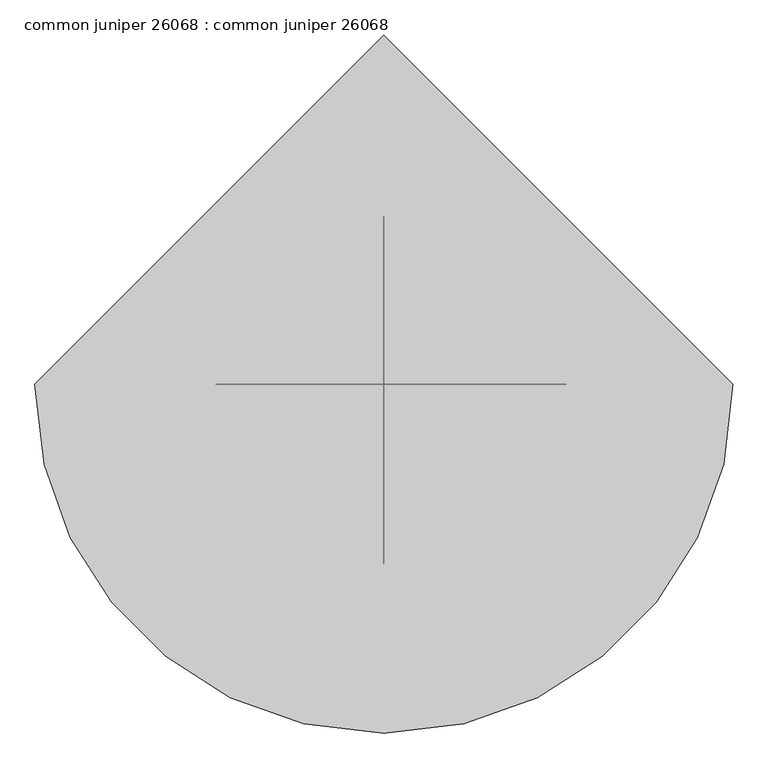
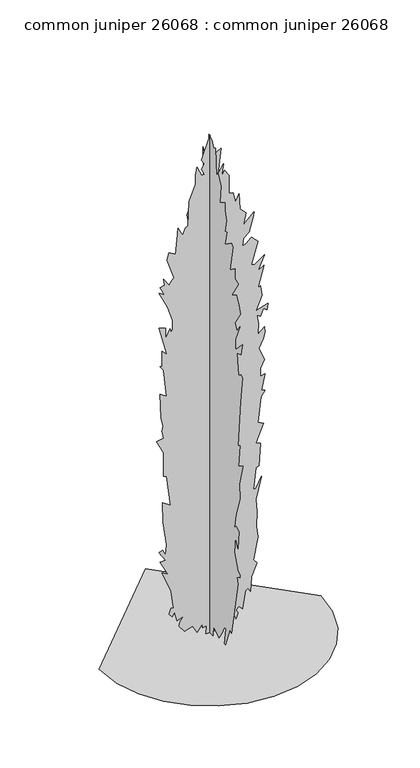
"""IFC4 building model written with IfcOpenShell, lengths in millimetres: proxy geometry, common juniper 26068 : common juniper 26068."""

from ifc_helpers import new_model, si_unit, origin, place, context, project, spatial, triangles, source, transform, mapped, element, save


def common_juniper_26068_common_juniper_26068_35e030ca(model_context):
    return source(origin(), model_context, "Body", "Tessellation", [
        triangles([(2e-06, 20.8572502, 34.4973742), (2.9e-06, 50.3272151, 21.867388), (4.9e-06, 67.1674663, 63.9673119), (4e-06, 75.5873421, 21.867388), (6e-06, 105.0572775, 42.9175021), (6.8e-06, 126.1073371, 38.7074393), (1.05e-05, 163.9974026, 106.0674356), (1.16e-05, 163.9974026, 143.9575011), (1.1e-05, 147.1574058, 148.1673096), (1.26e-05, 147.1574058, 202.8973719), (1.29e-05, 176.6273366, 169.2173783), (1.44e-05, 185.0474622, 207.1074347), (1.33e-05, 155.577277, 211.3174975), (1.5e-05, 155.577277, 270.2568686), (1.59e-05, 172.4172738, 274.4682032), (2.15e-05, 208.9710382, 408.6238226), (2.29e-05, 206.0972674, 459.7084588), (2.67e-05, 248.1971505, 522.8581289), (2.46e-05, 201.8872046, 522.8581289), (2.34e-05, 185.1554134, 508.0702234), (2.48e-05, 172.4172738, 573.376339), (2.87e-05, 210.3073302, 649.1574692), (2.78e-05, 174.6776373, 670.1633818), (3.35e-05, 214.5174112, 800.7172588), (3.23e-05, 197.6771419, 788.0883059), (3.52e-05, 206.0972674, 872.2870182), (4.35e-05, 239.7772792, 1099.6279381), (4.31e-05, 214.5174112, 1124.8883148), (4.64e-05, 221.6324747, 1223.064735), (4.69e-05, 206.0972674, 1263.816608), (5.28e-05, 239.7772792, 1411.1674976), (5.42e-05, 214.5174112, 1495.3662827), (5.6e-05, 239.7772792, 1520.6266594), (5.93e-05, 214.5174112, 1667.977549), (5.58e-05, 162.8142626, 1629.2094212), (5.8e-05, 189.2572706, 1663.7663235), (6.33e-05, 189.2572706, 1840.5863445), (6.26e-05, 176.6273366, 1836.3775898), (6.33e-05, 176.6273366, 1857.4265957), (6.27e-05, 163.9971482, 1857.4265957), (6.42e-05, 172.4172738, 1895.3184689), (6.36e-05, 159.7870854, 1895.3184689), (6.46e-05, 172.4172738, 1907.9474945), (6.6e-05, 184.4045872, 1938.4732475), (6.63e-05, 168.207211, 1971.0971283), (6.38e-05, 138.7372802, 1933.2078712), (6.66e-05, 147.1571514, 2013.1977562), (6.57e-05, 130.3171455, 2008.9863853), (6.57e-05, 113.4776574, 2034.2467621), (6.82e-05, 130.3171455, 2093.1876411), (6.79e-05, 117.6872115, 2101.6077667), (6.74e-05, 115.2719156, 2088.51656), (6.69e-05, 112.8578914, 2076.3093109), (6.65e-05, 110.4461564, 2065.872448), (6.62e-05, 108.0382274, 2058.0897835), (6.59e-05, 105.6348767, 2053.8454205), (6.58e-05, 103.2373577, 2054.0233166), (6.59e-05, 100.8472147, 2059.5071388), (6.74e-05, 67.167212, 2160.5486458), (6.91e-05, 79.797146, 2198.4380482), (6.81e-05, 50.3272151, 2211.0669285), (7.25e-05, 54.7259973, 2350.8028759), (6.92e-05, 29.2771487, 2278.4279331), (6.92e-05, 12.4371758, 2303.6883099), (7e-05, 12.4371758, 2328.9486866), (7.13e-05, 1.9569493, 2388.087664), (7.3e-05, 8.22762, 2438.4078484), (7.15e-05, -17.0328629, 2425.7763519), (7.01e-05, -29.662722, 2396.3072205), (6.96e-05, -46.5027211, 2404.727346), (6.53e-05, -54.9228512, 2274.2165623), (6.54e-05, -63.3427225, 2291.0568134), (6.29e-05, -89.9589621, 2244.0082317), (6.07e-05, -82.3490978, 2159.977169), (5.96e-05, -122.2828521, 2181.597797), (5.84e-05, -122.3656505, 2144.5212811), (5.66e-05, -134.9127861, 2101.6077667), (5.54e-05, -122.2828521, 2042.6668877), (5.48e-05, -138.0380133, 2047.4395615), (5.35e-05, -122.2828521, 1979.5172539), (5.23e-05, -172.8028426, 2013.1977562), (5.13e-05, -186.3878237, 2001.8109512), (4.87e-05, -163.5081882, 1878.2927639), (4.78e-05, -202.2725372, 1907.9474945), (4.63e-05, -202.2725372, 1857.4265957), (4.47e-05, -231.7427224, 1849.0064701), (4.47e-05, -177.0129054, 1764.8078304), (4.36e-05, -214.9027256, 1785.8568363), (4.15e-05, -235.9527852, 1747.9675793), (4e-05, -244.3729108, 1710.0783222), (3.99e-05, -202.2725372, 1642.7171722), (3.83e-05, -219.1127884, 1613.2480408), (3.83e-05, -241.2687761, 1646.3393349), (3.74e-05, -205.5590554, 1563.0676735), (3.58e-05, -206.4828544, 1512.2065338), (3.51e-05, -261.2118902, 1571.1474129), (3.4e-05, -248.5827192, 1512.2065338), (3.5e-05, -219.1127884, 1503.7864082), (3.14e-05, -231.7427224, 1402.7473721), (3.11e-05, -248.5827192, 1415.3763977), (3.03e-05, -261.2118902, 1406.9562721), (2.72e-05, -244.3729108, 1280.6568592), (2.12e-05, -227.5326596, 1053.3184828), (2.09e-05, -240.1625937, 1061.7386084), (1.81e-05, -231.7427224, 956.4883467), (1.73e-05, -265.4232247, 977.5373526), (1.54e-05, -237.9499925, 875.0023321), (1.31e-05, -240.1625937, 800.7172588), (1.16e-05, -210.6926628, 703.8870501), (1.01e-05, -198.0627288, 636.5285889), (9.9e-06, -210.6926628, 649.1574692), (8.4e-06, -235.9527852, 636.5285889), (6.2e-06, -227.5326596, 548.1185057), (8.5e-06, -206.4828544, 594.4279246), (6.5e-06, -198.0627288, 514.4380033), (2.9e-06, -227.5326596, 438.6568731), (2e-06, -243.3599639, 431.2197181), (1.5e-06, -243.5103181, 416.411465), (2.3e-06, -219.1127884, 404.9763708), (1e-06, -227.5326596, 375.5071667), (-4.7e-06, -172.8028426, 101.8573729), (-3.9e-06, -160.1726542, 110.2774984), (-5.1e-06, -126.4926606, 17.6574001), (-4.8e-06, -118.0727893, 17.6574001), (-2.9e-06, -130.7027234, 97.6473101), (-2.4e-06, -118.0727893, 97.6473101), (-2.7e-06, -97.022212, 55.5474361), (-2.7e-06, -71.7625937, 17.6574001), (1e-07, -29.662722, 47.1273105), (-1.2e-06, -26.985301, 2.08e-05), (1.1e-06, 25.0673653, 2.23e-05), (-515.3041569, -1e-07, 3.69e-05), (-501.6820959, -118.0735524, 3.3e-05), (-462.8834467, -226.5052332, 2.86e-05), (-402.0172491, -322.1873471, 2.4e-05), (-322.1873471, -402.0172491, 1.92e-05), (-226.5052332, -462.8834467, 1.45e-05), (-118.0735524, -501.6820959, 1.02e-05), (2.25e-05, -515.3041569, 6.2e-06), (118.0735524, -501.6820959, 3.1e-06), (226.5052332, -462.8834467, 1e-06), (322.1873471, -402.0172491, 0.0), (402.0172491, -322.1873471, 0.0), (462.8834467, -226.5052332, 1e-06), (501.6820959, -118.0735524, 3.1e-06), (515.3041569, 4.49e-05, 6.2e-06), (-6.76e-05, 515.3041569, 3.69e-05), (-18.1277839, 9e-07, 2.21e-05), (-15.9294828, -9e-07, 38.9106382), (-33.6886368, -1e-07, 34.4973742), (-33.6886368, -1.1e-06, 55.5474361), (-58.9485094, 1.2e-06, 21.8674629), (-79.998569, 1e-07, 59.7575034), (-117.8886345, 2.9e-06, 47.1273105), (-143.1485116, 2.2e-06, 80.8073133), (-138.9386941, 0.0, 101.8573729), (-122.098443, -1.5e-06, 122.9074415), (-151.5686372, 0.0, 110.2774984), (-164.1985713, -1.7e-06, 156.5874443), (-176.8285053, -6e-07, 139.7474384), (-189.4584393, -1e-06, 156.5874443), (-181.0385681, -2.3e-06, 181.8473123), (-168.4083797, -2.7e-06, 181.8473123), (-180.3558154, -7.3e-06, 266.0887183), (-223.1384511, -1.18e-05, 371.2983756), (-193.6685021, -1.19e-05, 354.4581244), (-231.5585767, -1.51e-05, 426.0279565), (-206.2984361, -1.59e-05, 426.0279565), (-236.2903554, -1.71e-05, 473.5007129), (-218.928897, -1.91e-05, 480.757501), (-206.2984361, -1.81e-05, 451.2883332), (-202.0883733, -2.05e-05, 501.8065433), (-216.5369645, -2.75e-05, 615.9519379), (-218.928897, -3.28e-05, 712.3071756), (-183.4688521, -3.28e-05, 688.38538), (-202.0883733, -4.12e-05, 838.6065159), (-214.7185799, -4.1e-05, 842.8178867), (-214.7185799, -4.73e-05, 956.4883467), (-248.3983191, -5.04e-05, 1023.8468079), (-214.7185799, -5.16e-05, 1028.058106), (-221.9263521, -5.3e-05, 1065.2057659), (-216.8864708, -5.54e-05, 1088.911659), (-227.3485139, -5.7e-05, 1133.3084404), (-231.5585767, -6.44e-05, 1251.1877277), (-202.0883733, -6.44e-05, 1230.1385765), (-214.7185799, -7.1e-05, 1360.6467442), (-231.5585767, -7.27e-05, 1385.9071209), (-223.1384511, -7.28e-05, 1381.6983662), (-223.1384511, -7.73e-05, 1457.4770256), (-199.0627223, -7.69e-05, 1431.8229229), (-235.7683851, -8.33e-05, 1575.3561676), (-205.5140908, -8.37e-05, 1563.9058491), (-206.2984361, -8.14e-05, 1512.2065338), (-185.2483765, -8.39e-05, 1554.3071617), (-181.0385681, -8.33e-05, 1537.4669106), (-172.6184425, -8.39e-05, 1545.8870361), (-172.4459785, -8.71e-05, 1592.2497585), (-195.9021957, -9.07e-05, 1663.7815842), (-235.7683851, -9.33e-05, 1747.9675793), (-210.5084989, -9.33e-05, 1731.1273281), (-231.5585767, -9.57e-05, 1773.227956), (-210.5084989, -9.65e-05, 1777.4367107), (-214.7185799, -9.77e-05, 1806.9084583), (-189.4584393, -9.68e-05, 1769.0165852), (-176.8285053, -9.92e-05, 1790.0682072), (-165.3669774, -9.99e-05, 1797.7949158), (-197.8783105, -0.0001044, 1895.3184689), (-189.4584393, -0.0001062, 1928.9965004), (-159.9885085, -0.0001063, 1912.1562492), (-151.5683829, -0.0001107, 1979.5172539), (-147.3585744, -0.0001144, 2034.2467621), (-126.3085057, -0.0001131, 1992.1461342), (-113.6788261, -0.000115, 2025.8266365), (-101.0483834, -0.0001167, 2030.0380074), (-96.8383206, -0.0001232, 2147.9172947), (-67.4105474, -0.0001297, 2222.3166779), (-67.3683806, -0.0001316, 2265.7964367), (-58.9482551, -0.0001347, 2303.6883099), (-37.8984453, -0.0001321, 2257.3763111), (-25.268484, -0.0001336, 2257.3763111), (-37.8984453, -0.0001346, 2286.8480587), (-25.268484, -0.0001359, 2307.8970646), (-37.8984453, -0.0001365, 2328.9462158), (-0.0084209, -0.0001447, 2438.4078484), (4.2015544, -0.0001387, 2324.7373158), (21.0416299, -0.0001399, 2341.5775669), (33.6716184, -0.0001405, 2345.786467), (50.5116198, -0.0001427, 2358.4178181), (37.8816812, -0.0001346, 2236.3273052), (63.1415538, -0.0001383, 2278.4279331), (54.7216826, -0.0001341, 2215.2782993), (67.3516166, -0.000137, 2244.7474308), (88.4014264, -0.000135, 2211.0669285), (88.4014264, -0.0001299, 2122.656918), (107.6572278, -0.0001303, 2118.4099388), (117.8716207, -0.0001285, 2072.1386353), (134.7116175, -0.0001316, 2105.8166668), (138.9216803, -0.0001272, 2030.0380074), (168.3916111, -0.0001268, 2000.5662598), (155.7614227, -0.0001229, 1945.8367516), (205.6238225, -0.0001275, 1992.2782482), (202.8546965, -0.0001267, 1974.4448891), (182.6657035, -0.0001205, 1900.3248493), (155.7614227, -0.0001187, 1878.4782177), (151.5516143, -0.000116, 1844.7977154), (168.3916111, -0.0001178, 1849.0064701), (193.6514973, -0.0001195, 1870.0580921), (223.1216825, -0.000119, 1840.5863445), (193.6514973, -0.0001114, 1739.5474537), (206.2816857, -0.0001114, 1731.1273281), (252.5916133, -0.0001165, 1764.8078304), (223.1216825, -0.0001104, 1697.4468258), (251.7186107, -0.000113, 1712.8392002), (223.1216825, -0.0001055, 1613.2480408), (235.7516165, -0.000106, 1617.4567955), (242.5560522, -0.0001041, 1569.0011776), (214.7015569, -9.92e-05, 1503.7864082), (269.4313558, -0.0001027, 1520.6266594), (265.2225647, -0.0001001, 1491.1575279), (248.3815506, -0.0001002, 1503.7864082), (235.7516165, -9.72e-05, 1470.1083767), (218.9116197, -9.71e-05, 1478.5285023), (225.9123915, -9.55e-05, 1438.523386), (223.1214282, -9.19e-05, 1385.9071209), (252.5916133, -9.51e-05, 1411.1674976), (256.8024392, -9.41e-05, 1385.9071209), (248.3815506, -9.14e-05, 1356.4379894), (227.3314909, -8.77e-05, 1314.3373615), (252.5916133, -8.56e-05, 1251.1877277), (235.7516165, -8.23e-05, 1213.298398), (235.7516165, -8.06e-05, 1175.4065248), (256.8024392, -8.14e-05, 1179.6178957), (239.961425, -7.64e-05, 1103.8367655), (256.8024392, -7.67e-05, 1099.6279381), (237.7775285, -7.39e-05, 1074.3497572), (223.1214282, -6.58e-05, 952.2769758), (248.3815506, -6.71e-05, 939.6480955), (214.7015569, -6.01e-05, 855.446767), (235.7513622, -6.03e-05, 847.0266415), (227.3314909, -5.4e-05, 737.5675524), (214.7015569, -5.23e-05, 733.3562542), (202.0711142, -4.63e-05, 632.317218), (214.7015569, -4.67e-05, 632.317218), (239.961425, -5.08e-05, 682.8379715), (214.7015569, -4.31e-05, 577.5876735), (218.9116197, -4.06e-05, 518.6467944), (216.6522736, -3.6e-05, 443.0028288), (223.1214282, -3.28e-05, 392.3474178), (202.0711142, -2.52e-05, 287.0971198), (218.9116197, -2.48e-05, 266.0480776), (193.6514973, -2.03e-05, 207.1074347), (189.4414345, -1.58e-05, 135.5373756), (176.8114823, -1.64e-05, 156.5874443), (164.1815483, -1.56e-05, 148.1673096), (151.5513599, -1.04e-05, 63.9673119), (134.7116175, -1.06e-05, 80.8073133), (122.0814291, -9.7e-06, 68.1773747), (130.5015547, -8e-06, 51.3373733), (122.0814291, -6.7e-06, 26.0775007), (113.6615579, -7.2e-06, 42.9172477), (75.7714924, -5.9e-06, 38.7074393), (71.561425, -3.1e-06, 5.0273616), (63.1415538, -3.8e-06, 26.0775007), (50.5113654, -4e-06, 38.7074393), (16.5476705, -2.2e-06, 20.6906271), (21.2391151, -2e-07, 2.1e-05)], [[92, 93, 94], [61, 62, 63], [112, 113, 114], [95, 96, 97], [95, 97, 98], [23, 24, 25], [105, 106, 107], [103, 104, 105], [83, 84, 85], [10, 11, 12], [10, 12, 13], [71, 72, 73], [17, 18, 19], [17, 19, 20], [66, 67, 68], [66, 68, 69], [78, 79, 80], [74, 75, 76], [33, 34, 35], [44, 45, 46], [43, 44, 46], [3, 4, 5], [50, 51, 52], [49, 50, 52], [49, 52, 53], [49, 53, 54], [49, 54, 55], [49, 55, 56], [69, 70, 71], [120, 121, 122], [46, 47, 48], [36, 37, 38], [85, 86, 87], [40, 41, 42], [123, 124, 125], [122, 123, 125], [111, 112, 114], [110, 111, 114], [42, 43, 46], [130, 131, 1], [129, 130, 1], [66, 69, 71], [65, 66, 71], [64, 65, 71], [1, 2, 3], [127, 128, 129], [87, 88, 89], [38, 39, 40], [21, 22, 23], [59, 60, 61], [32, 33, 35], [63, 64, 71], [83, 85, 87], [7, 8, 9], [61, 63, 71], [80, 81, 82], [80, 82, 83], [5, 6, 7], [3, 5, 7], [3, 7, 9], [61, 71, 73], [61, 73, 74], [59, 61, 74], [58, 59, 74], [99, 100, 101], [99, 101, 102], [117, 118, 119], [116, 117, 119], [49, 56, 57], [87, 89, 90], [87, 90, 91], [14, 15, 16], [126, 127, 129], [26, 27, 28], [74, 76, 77], [58, 74, 77], [58, 77, 78], [58, 78, 80], [57, 58, 80], [49, 57, 80], [48, 49, 80], [46, 48, 80], [46, 80, 83], [46, 83, 87], [42, 46, 87], [40, 42, 87], [38, 40, 87], [36, 38, 87], [35, 36, 87], [35, 87, 91], [32, 35, 91], [32, 91, 92], [32, 92, 94], [32, 94, 95], [31, 32, 95], [30, 31, 95], [30, 95, 98], [30, 98, 99], [30, 99, 102], [30, 102, 103], [29, 30, 103], [28, 29, 103], [26, 28, 103], [26, 103, 105], [26, 105, 107], [25, 26, 107], [25, 107, 108], [25, 108, 109], [23, 25, 109], [23, 109, 110], [21, 23, 110], [21, 110, 114], [21, 114, 115], [20, 21, 115], [20, 115, 116], [20, 116, 119], [17, 20, 119], [16, 17, 119], [14, 16, 119], [14, 119, 120], [14, 120, 122], [14, 122, 125], [14, 125, 126], [13, 14, 126], [10, 13, 126], [10, 126, 129], [9, 10, 129], [3, 9, 129], [1, 3, 129], [146, 147, 132], [145, 146, 132], [145, 132, 133], [144, 145, 133], [144, 133, 134], [144, 134, 135], [143, 144, 135], [142, 143, 135], [142, 135, 136], [142, 136, 137], [142, 137, 138], [142, 138, 139], [142, 139, 140], [142, 140, 141], [283, 284, 285], [223, 224, 225], [229, 230, 231], [202, 203, 204], [301, 302, 303], [236, 237, 238], [186, 187, 188], [250, 251, 252], [210, 211, 212], [198, 199, 200], [291, 292, 293], [217, 218, 219], [164, 165, 166], [240, 241, 242], [193, 194, 195], [188, 189, 190], [240, 242, 243], [298, 299, 300], [252, 253, 254], [227, 228, 229], [183, 184, 185], [222, 223, 225], [294, 295, 296], [173, 174, 175], [231, 232, 233], [264, 265, 266], [258, 259, 260], [257, 258, 260], [166, 167, 168], [151, 152, 153], [271, 272, 273], [273, 274, 275], [257, 260, 261], [257, 261, 262], [178, 179, 180], [159, 160, 161], [159, 161, 162], [159, 162, 163], [226, 227, 229], [225, 226, 229], [264, 266, 267], [216, 217, 219], [207, 208, 209], [200, 201, 202], [200, 202, 204], [149, 150, 151], [305, 306, 148], [305, 148, 149], [254, 255, 256], [168, 169, 170], [168, 170, 171], [222, 225, 229], [221, 222, 229], [220, 221, 229], [157, 158, 159], [297, 298, 300], [282, 283, 285], [301, 303, 304], [276, 277, 278], [246, 247, 248], [246, 248, 249], [245, 246, 249], [206, 207, 209], [231, 233, 234], [240, 243, 244], [278, 279, 280], [278, 280, 281], [153, 154, 155], [153, 155, 156], [153, 156, 157], [176, 177, 178], [191, 192, 193], [190, 191, 193], [264, 267, 268], [297, 300, 301], [234, 235, 236], [289, 290, 291], [238, 239, 240], [304, 305, 149], [209, 210, 212], [151, 153, 157], [212, 213, 214], [190, 193, 195], [216, 219, 220], [216, 220, 229], [215, 216, 229], [215, 229, 231], [215, 231, 234], [214, 215, 234], [214, 234, 236], [214, 236, 238], [214, 238, 240], [212, 214, 240], [212, 240, 244], [209, 212, 244], [206, 209, 244], [206, 244, 245], [206, 245, 249], [186, 188, 190], [254, 256, 257], [268, 269, 270], [205, 206, 249], [204, 205, 249], [200, 204, 249], [198, 200, 249], [197, 198, 249], [196, 197, 249], [196, 249, 250], [196, 250, 252], [196, 252, 254], [196, 254, 257], [196, 257, 262], [196, 262, 263], [196, 263, 264], [195, 196, 264], [190, 195, 264], [186, 190, 264], [185, 186, 264], [185, 264, 268], [185, 268, 270], [185, 270, 271], [183, 185, 271], [182, 183, 271], [182, 271, 273], [182, 273, 275], [182, 275, 276], [181, 182, 276], [180, 181, 276], [178, 180, 276], [176, 178, 276], [176, 276, 278], [175, 176, 278], [175, 278, 281], [175, 281, 282], [173, 175, 282], [172, 173, 282], [172, 282, 285], [172, 285, 286], [172, 286, 287], [171, 172, 287], [168, 171, 287], [166, 168, 287], [166, 287, 288], [166, 288, 289], [164, 166, 289], [164, 289, 291], [163, 164, 291], [163, 291, 293], [163, 293, 294], [163, 294, 296], [159, 163, 296], [157, 159, 296], [151, 157, 296], [151, 296, 297], [151, 297, 301], [151, 301, 304], [151, 304, 149]], closed=False),
    ])


if __name__ == "__main__":
    model = new_model("IFC4")
    model_context = context("Model", 3, world=origin())
    ifc_project = project(units=[si_unit("LENGTHUNIT", "METRE", prefix="MILLI")], contexts=[model_context])
    site = spatial("IfcSite", under=ifc_project)
    building = spatial("IfcBuilding", under=site)
    placement = place(None, origin())
    common_juniper_26068_common_juniper_26068_shape = common_juniper_26068_common_juniper_26068_35e030ca(model_context)
    element("IfcBuildingElementProxy", 1, Name="common juniper 26068 : common juniper 26068", ObjectType="common juniper 26068 : common juniper 26068", at=placement, inside=building, context=model_context, shape_type="MappedRepresentation", body=[
        mapped(common_juniper_26068_common_juniper_26068_shape, transform((0.0, 0.0, 0.0), x_axis=(1.0, 0.0, 0.0), y_axis=(0.0, 1.0, 0.0), z_axis=(0.0, 0.0, 1.0))),
    ])
    save(model, "model.ifc")

# Revit data of these elements
# Type "common juniper 26068 : common juniper 26068"
#   built-in parameter 1005195 = "RPC-16-G3GW-Q1G0-PMP1-8000-ST1L-LVER-AU"
#   Height = 0
